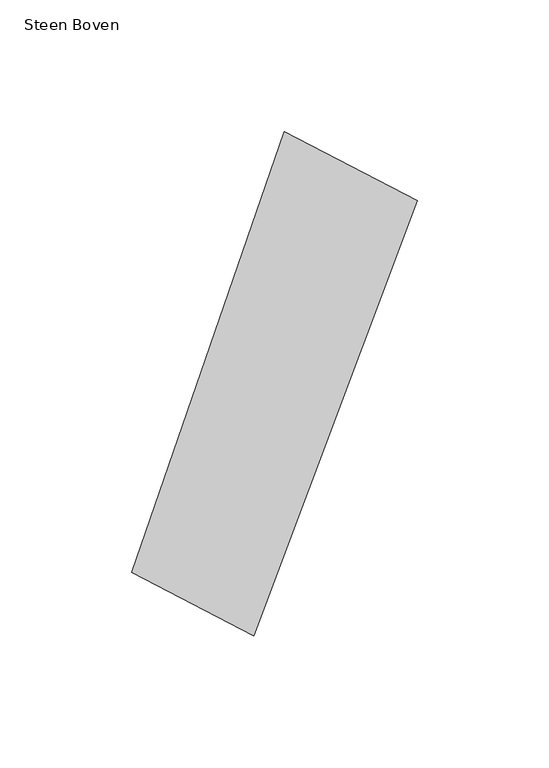
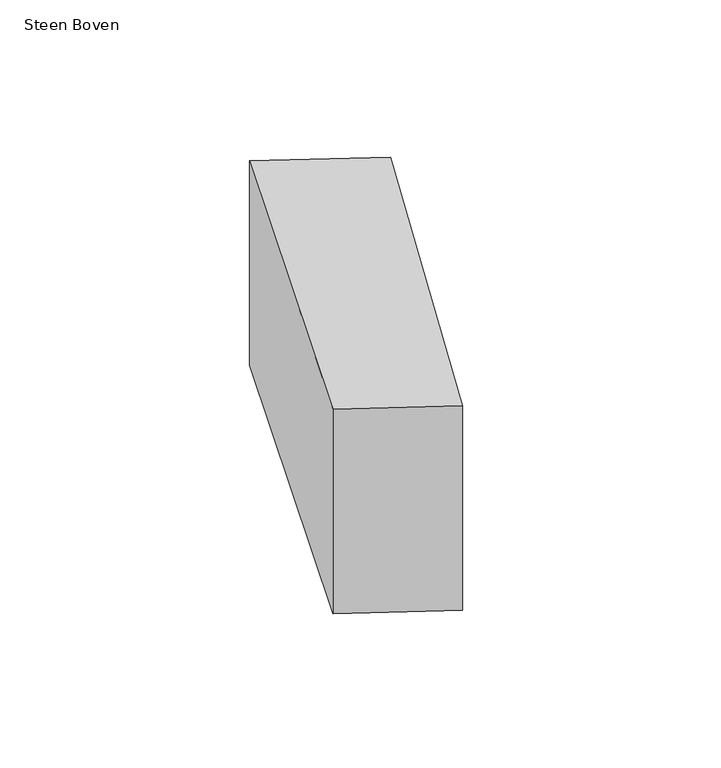
"""IFC4 building model written with IfcOpenShell, lengths in millimetres: proxy geometry, 00_GMA_steen_versie_4 : Steen Boven."""

from ifc_helpers import new_model, si_unit, origin, origin_with_axes, place, context, project, spatial, polyline, outline, extrude, source, transform, mapped, element, save


def steen_boven_009ee860(model_context):
    return source(origin(), model_context, "Body", "SweptSolid", [
        extrude(outline(polyline([(132.9592776, 155.7659209), (71.0255673, -9.2896775), (24.8598773, 14.6345055), (82.6544216, 181.8529402), (132.9592776, 155.7659209)])), origin_with_axes(), (0.0, 0.0, 1.0), 100.0),
    ])


if __name__ == "__main__":
    model = new_model("IFC4")
    model_context = context("Model", 3, world=origin())
    ifc_project = project(units=[si_unit("LENGTHUNIT", "METRE", prefix="MILLI")], contexts=[model_context])
    site = spatial("IfcSite", under=ifc_project)
    building = spatial("IfcBuilding", under=site)
    placement = place(None, origin())
    steen_boven_shape = steen_boven_009ee860(model_context)
    element("IfcBuildingElementProxy", 1, Name="00_GMA_steen_versie_4 : Steen Boven", ObjectType="00_GMA_steen_versie_4 : Steen Boven", at=placement, inside=building, context=model_context, shape_type="MappedRepresentation", body=[
        mapped(steen_boven_shape, transform((0.0, 0.0, 0.0), x_axis=(1.0, 0.0, 0.0), y_axis=(0.0, 1.0, 0.0), z_axis=(0.0, 0.0, 1.0))),
    ])
    save(model, "model.ifc")

# Revit data of these elements
# Type "00_GMA_steen_versie_4 : Steen Boven"
#   StootVoegHalfBoven [instance default] = 5 mm
#   StootVoegHalf [instance default] = 5 mm
#   StootVoegBreedteOnder = 10 mm
#   StootVoegBreedteBoven = 10 mm
#   Steendikte = 100 mm
#   LintVoegOnderHalf = 5 mm
#   LintVoegOnder = 10 mm
#   LintVoegBovenHalf = 0 mm
#   LintVoegBoven = 0 mm
#   materiaal = none
#   MateriaalVoeg = none
#   Default Elevation = 0
